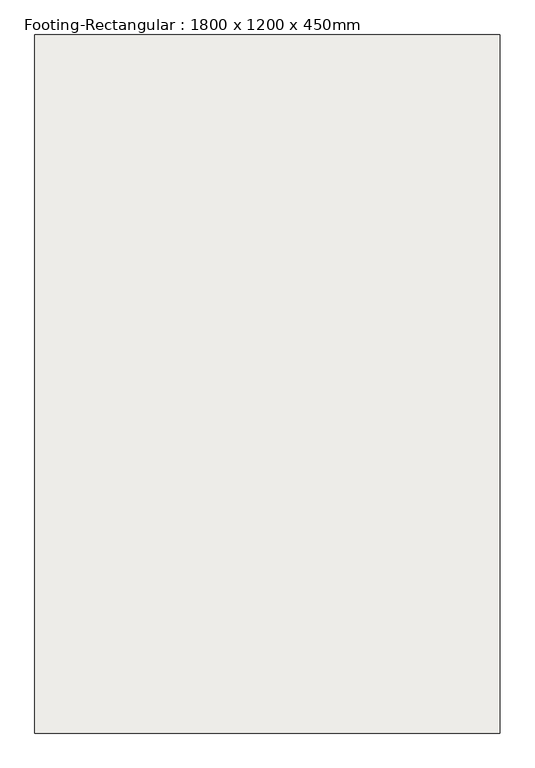
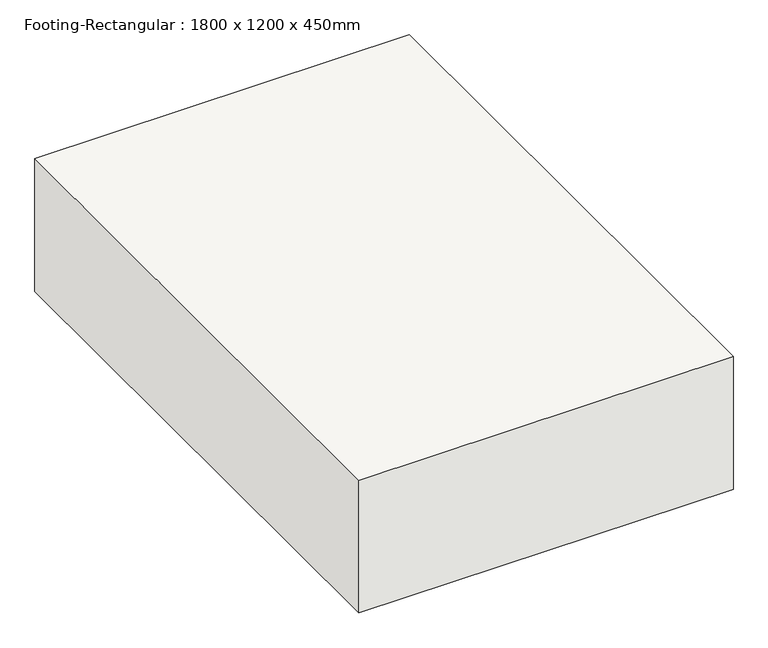
"""IFC4 building model written with IfcOpenShell, lengths in millimetres: slab geometry, Footing-Rectangular : 1800 x 1200 x 450mm."""

from ifc_helpers import new_model, si_unit, frame, origin, place, context, project, spatial, polyline, outline, extrude, source, transform, mapped, element, save


def footing_rectangular_1800_x_1200_x_450mm_16ba7ea5(model_context):
    return source(origin(), model_context, "Body", "SweptSolid", [
        extrude(outline(polyline([(600.0, 900.0), (600.0, -900.0), (-600.0, -900.0), (-600.0, 900.0), (600.0, 900.0)])), frame((0.0, 0.0, -450.0), z_axis=(0.0, 0.0, 1.0), x_axis=(1.0, 0.0, 0.0)), (0.0, 0.0, 1.0), 450.0),
    ])


if __name__ == "__main__":
    model = new_model("IFC4")
    model_context = context("Model", 3, world=origin())
    ifc_project = project(units=[si_unit("LENGTHUNIT", "METRE", prefix="MILLI")], contexts=[model_context])
    site = spatial("IfcSite", under=ifc_project)
    building = spatial("IfcBuilding", under=site)
    placement = place(None, origin())
    footing_rectangular_1800_x_1200_x_450mm_shape = footing_rectangular_1800_x_1200_x_450mm_16ba7ea5(model_context)
    element("IfcSlab", 1, ObjectType="Footing-Rectangular : 1800 x 1200 x 450mm", at=placement, inside=building, context=model_context, shape_type="MappedRepresentation", body=[
        mapped(footing_rectangular_1800_x_1200_x_450mm_shape, transform((0.0, 0.0, 0.0), x_axis=(1.0, 0.0, 0.0), y_axis=(0.0, 1.0, 0.0), z_axis=(0.0, 0.0, 1.0))),
    ])
    save(model, "model.ifc")

# Revit data of these elements
# Type "Footing-Rectangular : 1800 x 1200 x 450mm"
#   Width = 1200 mm
#   Length = 1800 mm
#   Foundation Thickness = 450 mm
#   Structural Material [instance default] = Concrete - Cast-in-Place Concrete
#   Assembly Code = ""
# Element 1 (IfcSlab, "Footing-Rectangular : 1800 x 1200 x 450mm")
#   Materials on its faces: "Concrete - Cast-in-Place Concrete"
# Materials
#   "Concrete - Cast-in-Place Concrete": class "Concrete", colour RGB 192 192 192, transparency 0, Cost = 0
